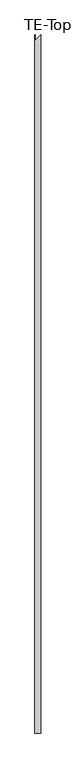
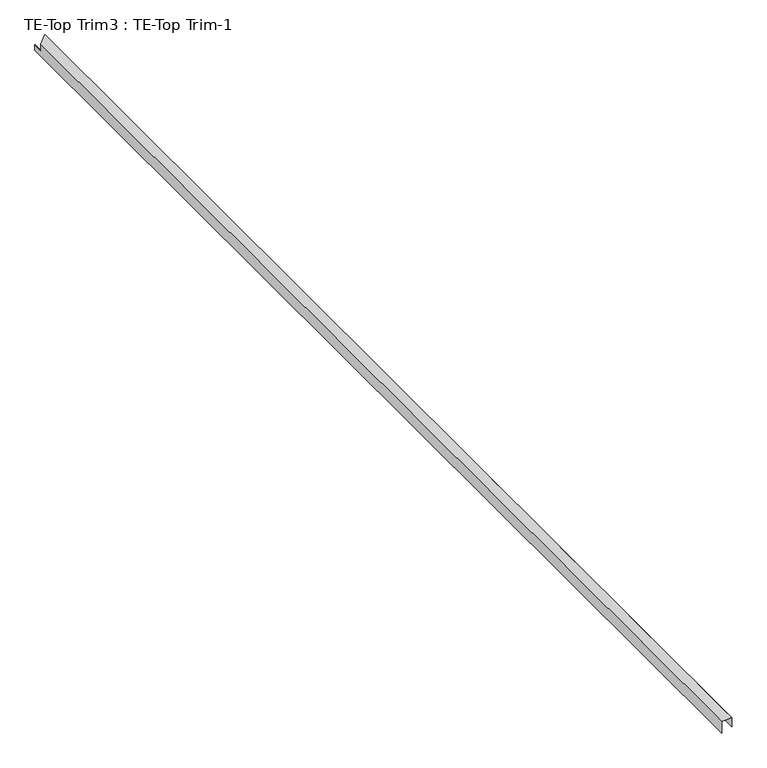
"""IFC4 building model written with IfcOpenShell, lengths in millimetres: proxy geometry, TE-Top Trim3 : TE-Top Trim-1."""

from ifc_helpers import new_model, si_unit, origin, place, context, project, spatial, faceted_brep, source, transform, mapped, element, save


def te_top_trim3_te_top_trim_1_5eaecf50(model_context):
    return source(origin(), model_context, "Body", "Brep", [
        faceted_brep([(590352.6755052, -531600.3289841, 2387.6), (590351.7825364, -531600.3289841, 2387.6), (590351.7825364, -531600.3289841, 2411.4125), (590352.6755052, -531600.3289841, 2411.4125), (590393.3931339, -531600.3289841, 2439.2929688), (590393.3931339, -531600.3289841, 2400.3), (590392.4558739, -531600.3289841, 2400.3), (590392.4558739, -531600.3289841, 2411.4125), (590392.4558739, -531600.3289841, 2438.4), (590392.4459322, -531600.3289841, 2439.2929688), (590352.6755052, -536420.7663841, 2387.6), (590352.6755052, -536420.7663841, 2438.4), (590392.4558739, -536420.7663841, 2438.4), (590392.4558739, -536420.7663841, 2400.3), (590393.3931339, -536420.7663841, 2400.3), (590393.3931339, -536420.7663841, 2439.2929688), (590351.7825364, -536420.7663841, 2439.2929688), (590351.7825364, -536420.7663841, 2387.6), (590351.7825364, -531640.9923799, 2439.2929688), (590351.7825364, -531640.9923799, 2411.4125), (590352.6755052, -531640.0994112, 2438.4), (590352.6755052, -531640.0994112, 2411.4125)], [[[0, 1, 2, 3]], [[4, 5, 6, 7, 8, 9]], [[10, 11, 12, 13, 14, 15, 16, 17]], [[1, 0, 10, 17]], [[17, 16, 18, 19, 2, 1]], [[16, 15, 4, 9, 18]], [[5, 4, 15, 14]], [[6, 5, 14, 13]], [[13, 12, 8, 7, 6]], [[12, 11, 20, 8]], [[11, 10, 0, 3, 21, 20]], [[19, 21, 3, 2]], [[21, 19, 18, 9, 8, 20]]]),
    ])


if __name__ == "__main__":
    model = new_model("IFC4")
    model_context = context("Model", 3, world=origin())
    ifc_project = project(units=[si_unit("LENGTHUNIT", "METRE", prefix="MILLI")], contexts=[model_context])
    site = spatial("IfcSite", under=ifc_project)
    building = spatial("IfcBuilding", under=site)
    placement = place(None, origin())
    te_top_trim3_te_top_trim_1_shape = te_top_trim3_te_top_trim_1_5eaecf50(model_context)
    element("IfcBuildingElementProxy", 1, Name="TE-Top Trim3 : TE-Top Trim-1", ObjectType="TE-Top Trim3 : TE-Top Trim-1", at=placement, inside=building, context=model_context, shape_type="MappedRepresentation", body=[
        mapped(te_top_trim3_te_top_trim_1_shape, transform((0.0, 0.0, 0.0), x_axis=(1.0, 0.0, 0.0), y_axis=(0.0, 1.0, 0.0), z_axis=(0.0, 0.0, 1.0))),
    ])
    save(model, "model.ifc")

# Revit data of these elements
# Element 1 (IfcBuildingElementProxy, "TE-Top Trim3 : TE-Top Trim-1")
#   Materials on its faces: "EDGE TRIM BY MTL PANEL MFR."
# Materials
#   "EDGE TRIM BY MTL PANEL MFR.": class "Generic", colour RGB 239 242 240, transparency 0, Cost = 0
